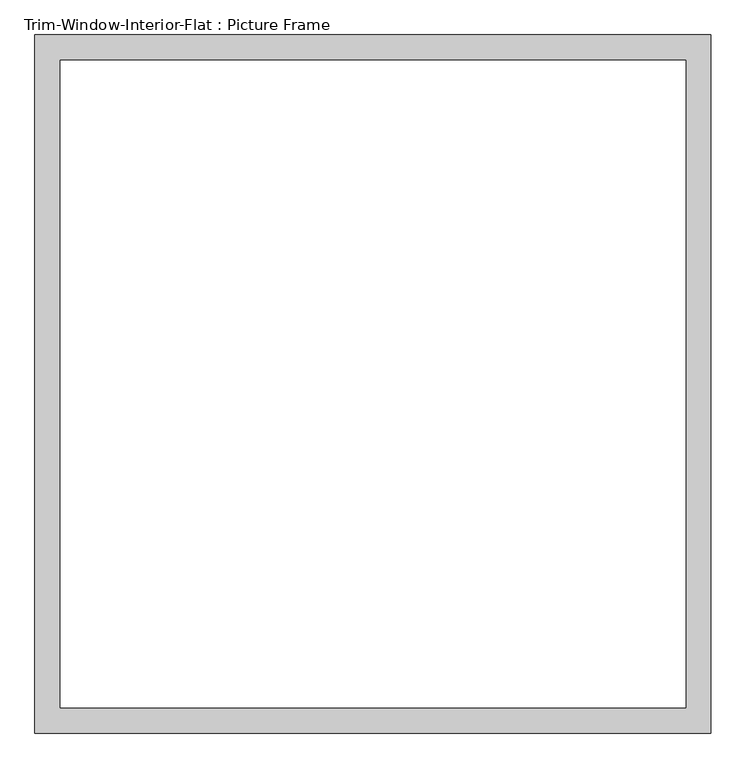
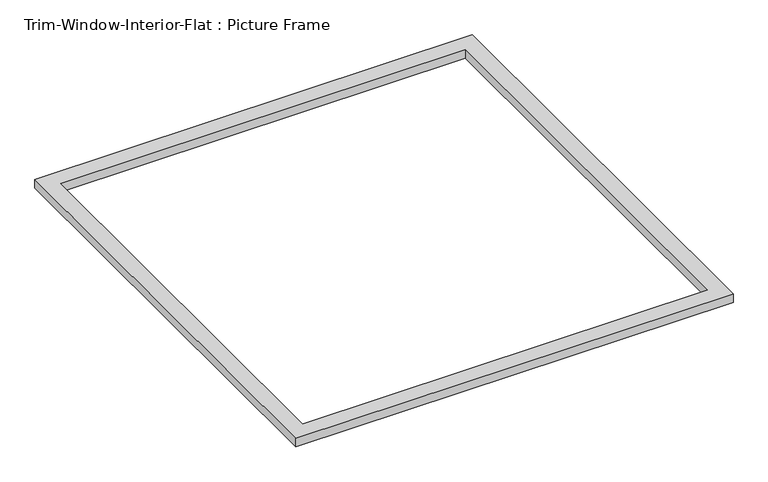
"""IFC4 building model written with IfcOpenShell, lengths in millimetres: proxy geometry, Trim-Window-Interior-Flat : Picture Frame."""

from ifc_helpers import new_model, si_unit, origin, origin_with_axes, place, context, project, spatial, polyline, outline, extrude, source, transform, mapped, element, save


def trim_window_interior_flat_picture_frame_59531e77(model_context):
    return source(origin(), model_context, "Body", "SweptSolid", [
        extrude(outline(polyline([(768.35, -44.45), (-768.35, -44.45), (-768.35, 1543.05), (768.35, 1543.05), (768.35, -44.45)]), holes=[polyline([(711.2, 12.7), (711.2, 1485.9), (-711.2, 1485.9), (-711.2, 12.7), (711.2, 12.7)])]), origin_with_axes(), (0.0, 0.0, 1.0), 31.75),
    ])


if __name__ == "__main__":
    model = new_model("IFC4")
    model_context = context("Model", 3, world=origin())
    ifc_project = project(units=[si_unit("LENGTHUNIT", "METRE", prefix="MILLI")], contexts=[model_context])
    site = spatial("IfcSite", under=ifc_project)
    building = spatial("IfcBuilding", under=site)
    placement = place(None, origin())
    trim_window_interior_flat_picture_frame_shape = trim_window_interior_flat_picture_frame_59531e77(model_context)
    element("IfcBuildingElementProxy", 1, Name="Trim-Window-Interior-Flat : Picture Frame", ObjectType="Trim-Window-Interior-Flat : Picture Frame", at=placement, inside=building, context=model_context, shape_type="MappedRepresentation", body=[
        mapped(trim_window_interior_flat_picture_frame_shape, transform((0.0, 0.0, 0.0), x_axis=(1.0, 0.0, 0.0), y_axis=(0.0, 1.0, 0.0), z_axis=(0.0, 0.0, 1.0))),
    ])
    save(model, "model.ifc")

# Revit data of these elements
# Type "Trim-Window-Interior-Flat : Picture Frame"
#   Trim Thickness_Picture Frame = 0' - 1 1/4"
#   Trim Width = 0' - 2 1/4"
#   Trim Thickness_with Sill = 0' - 0 3/4"
#   Sill Thickness = 0' - 1 1/4"
#   Opening Width [instance default] = 2' - 0"
#   Opening Height [instance default] = 3' - 0"
#   Default Elevation = 4' - 0"
#   Sill = no
#   Picture Frame = yes
#   Trim Material [instance default] = none
# Element 1 (IfcBuildingElementProxy, "Trim-Window-Interior-Flat : Picture Frame")
#   Opening Width = 4' - 9"
#   Opening Height = 4' - 11"
#   Trim Material = Wood - Stained
#   Materials on its faces: "Wood - Stained"
# Materials
#   "Wood - Stained": class "Wood", colour RGB 224 178 126, transparency 0, Cost = 0
